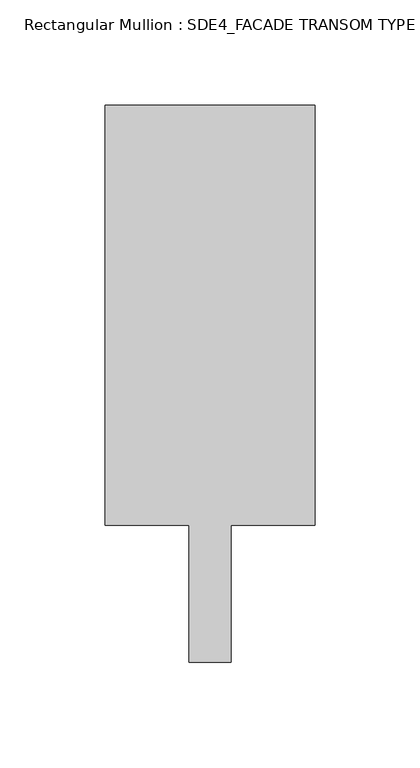
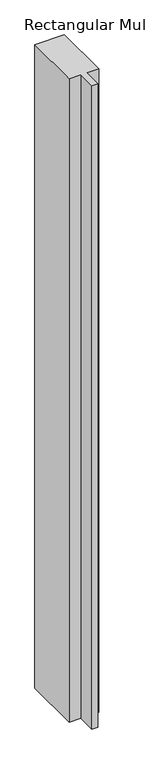
"""IFC4 building model written with IfcOpenShell, lengths in millimetres: member geometry, Rectangular Mullion : SDE4_FACADE TRANSOM TYPE 2."""

from ifc_helpers import new_model, si_unit, frame, origin, place, context, project, spatial, polyline, outline, extrude, source, transform, mapped, element, save


def rectangular_mullion_sde4_facade_transom_type_2_4e623b8d(model_context):
    return source(origin(), model_context, "Body", "SweptSolid", [
        extrude(outline(polyline([(50.0, 132.5), (50.0, -67.5), (10.0, -67.5), (10.0, -132.5), (-10.0, -132.5), (-10.0, -67.5), (-50.0, -67.5), (-50.0, 132.5), (50.0, 132.5)])), frame((0.0, 0.0, -2300.0), z_axis=(0.0, 0.0, 1.0), x_axis=(1.0, 0.0, 0.0)), (0.0, 0.0, 1.0), 2300.0),
    ])


if __name__ == "__main__":
    model = new_model("IFC4")
    model_context = context("Model", 3, world=origin())
    ifc_project = project(units=[si_unit("LENGTHUNIT", "METRE", prefix="MILLI")], contexts=[model_context])
    site = spatial("IfcSite", under=ifc_project)
    building = spatial("IfcBuilding", under=site)
    placement = place(None, origin())
    rectangular_mullion_sde4_facade_transom_type_2_shape = rectangular_mullion_sde4_facade_transom_type_2_4e623b8d(model_context)
    element("IfcMember", 1, ObjectType="Rectangular Mullion : SDE4_FACADE TRANSOM TYPE 2", at=placement, inside=building, context=model_context, shape_type="MappedRepresentation", body=[
        mapped(rectangular_mullion_sde4_facade_transom_type_2_shape, transform((0.0, 0.0, 0.0), x_axis=(1.0, 0.0, 0.0), y_axis=(0.0, 1.0, 0.0), z_axis=(0.0, 0.0, 1.0))),
    ])
    save(model, "model.ifc")

# Revit data of these elements
# Type "Rectangular Mullion : SDE4_FACADE TRANSOM TYPE 2"
#   built-in parameter 1007322 = 0.869423 (stored number, unit not read)
#   built-in parameter 1007321 = 0.164042 (stored number, unit not read)
#   built-in parameter 1007320 = 0.164042 (stored number, unit not read)
